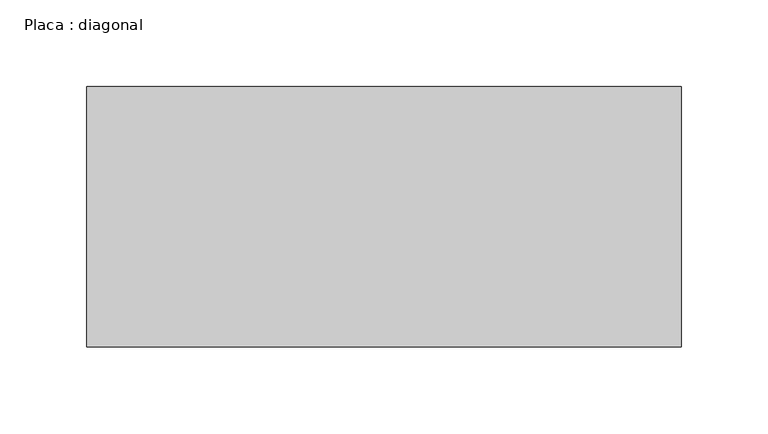
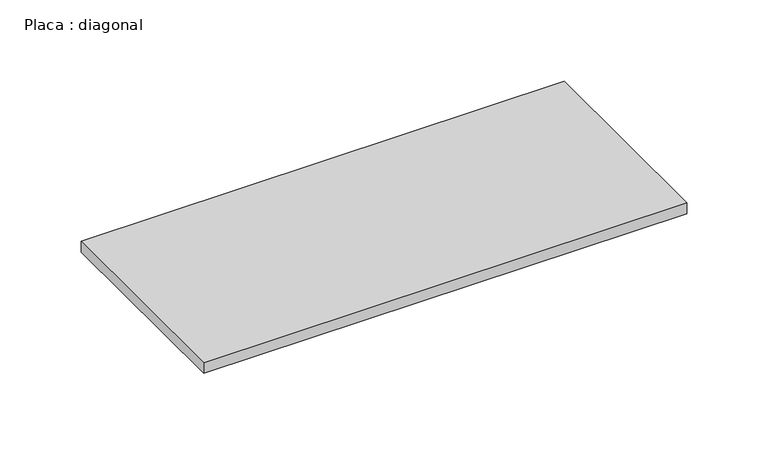
"""IFC4 building model written with IfcOpenShell, lengths in millimetres: beam geometry, Placa : diagonal."""

from ifc_helpers import new_model, si_unit, frame, origin, place, context, project, spatial, polyline, outline, extrude, source, transform, mapped, element, save


def placa_diagonal_c2548c1e(model_context):
    return source(origin(), model_context, "Body", "SweptSolid", [
        extrude(outline(polyline([(170.5911963, 75.0), (170.5911963, -75.0), (-171.5016566, -75.0), (-171.5016566, 75.0), (170.5911963, 75.0)])), frame((0.0, 0.0, -4.0), z_axis=(0.0, 0.0, 1.0), x_axis=(1.0, 0.0, 0.0)), (0.0, 0.0, 1.0), 8.0),
    ])


if __name__ == "__main__":
    model = new_model("IFC4")
    model_context = context("Model", 3, world=origin())
    ifc_project = project(units=[si_unit("LENGTHUNIT", "METRE", prefix="MILLI")], contexts=[model_context])
    site = spatial("IfcSite", under=ifc_project)
    building = spatial("IfcBuilding", under=site)
    placement = place(None, origin())
    placa_diagonal_shape = placa_diagonal_c2548c1e(model_context)
    element("IfcBeam", 1, ObjectType="Placa : diagonal", at=placement, inside=building, context=model_context, shape_type="MappedRepresentation", body=[
        mapped(placa_diagonal_shape, transform((0.0, 0.0, 0.0), x_axis=(1.0, 0.0, 0.0), y_axis=(0.0, 1.0, 0.0), z_axis=(0.0, 0.0, 1.0))),
    ])
    save(model, "model.ifc")

# Revit data of these elements
# Type "Placa : diagonal"
#   W = 0
#   Length [instance default] = 1.50 m
#   b = 0.15 m
#   d = 0.008 m
#   A = 0 m²
#   Structural Material [instance default] = Aço, 45-345
# Element 1 (IfcBeam, "Placa : diagonal")
#   Materials on its faces: "Aço, 45-345"
# Materials
#   "Aço, 45-345": class "Metal", colour RGB 247 247 247, transparency 0, Description = "Aço 345 MPa", Cost = 0
